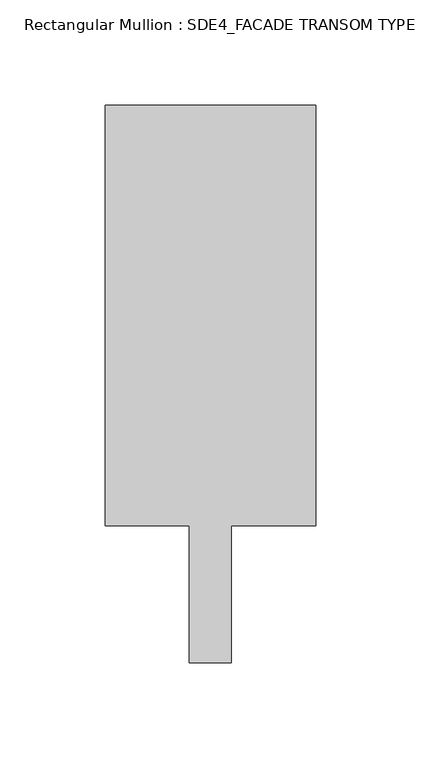
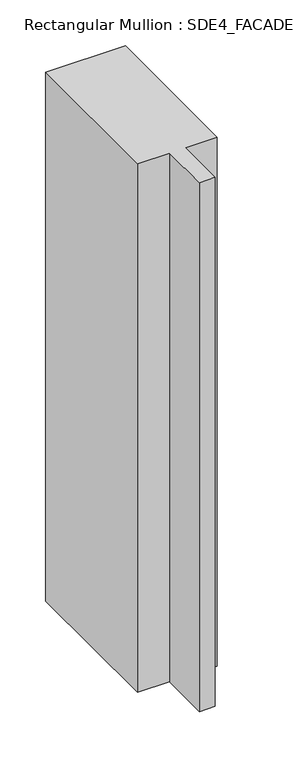
"""IFC4 building model written with IfcOpenShell, lengths in millimetres: member geometry, Rectangular Mullion : SDE4_FACADE TRANSOM TYPE 2."""

from ifc_helpers import new_model, si_unit, frame, origin, place, context, project, spatial, polyline, outline, extrude, source, transform, mapped, element, save


def rectangular_mullion_sde4_facade_transom_type_2_647f019d(model_context):
    return source(origin(), model_context, "Body", "SweptSolid", [
        extrude(outline(polyline([(50.0, 132.5), (50.0, -67.5), (10.0, -67.5), (10.0, -132.5), (-10.0, -132.5), (-10.0, -67.5), (-50.0, -67.5), (-50.0, 132.5), (50.0, 132.5)])), frame((0.0, 0.0, -702.372859), z_axis=(0.0, 0.0, 1.0), x_axis=(1.0, 0.0, 0.0)), (0.0, 0.0, 1.0), 702.372859),
    ])


if __name__ == "__main__":
    model = new_model("IFC4")
    model_context = context("Model", 3, world=origin())
    ifc_project = project(units=[si_unit("LENGTHUNIT", "METRE", prefix="MILLI")], contexts=[model_context])
    site = spatial("IfcSite", under=ifc_project)
    building = spatial("IfcBuilding", under=site)
    placement = place(None, origin())
    rectangular_mullion_sde4_facade_transom_type_2_shape = rectangular_mullion_sde4_facade_transom_type_2_647f019d(model_context)
    element("IfcMember", 1, ObjectType="Rectangular Mullion : SDE4_FACADE TRANSOM TYPE 2", at=placement, inside=building, context=model_context, shape_type="MappedRepresentation", body=[
        mapped(rectangular_mullion_sde4_facade_transom_type_2_shape, transform((0.0, 0.0, 0.0), x_axis=(1.0, 0.0, 0.0), y_axis=(0.0, 1.0, 0.0), z_axis=(0.0, 0.0, 1.0))),
    ])
    save(model, "model.ifc")

# Revit data of these elements
# Type "Rectangular Mullion : SDE4_FACADE TRANSOM TYPE 2"
#   built-in parameter 1007322 = 0.869423 (stored number, unit not read)
#   built-in parameter 1007321 = 0.164042 (stored number, unit not read)
#   built-in parameter 1007320 = 0.164042 (stored number, unit not read)
